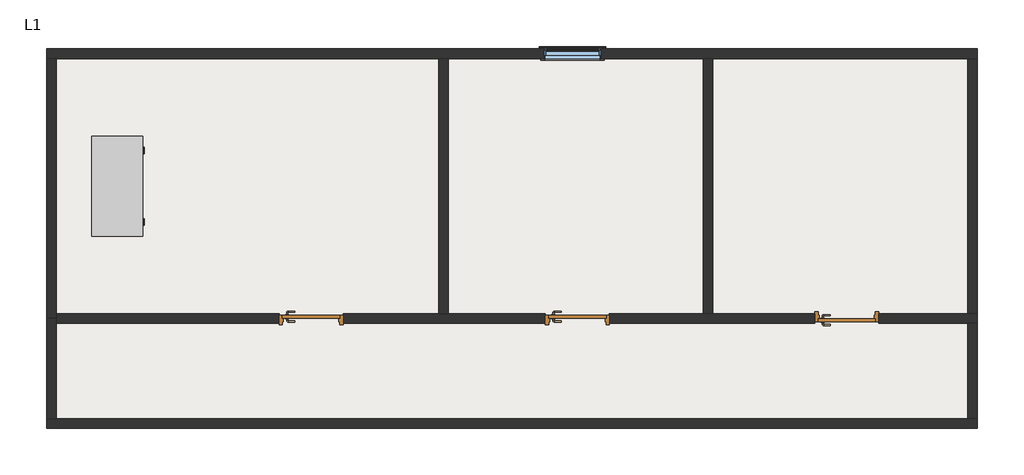
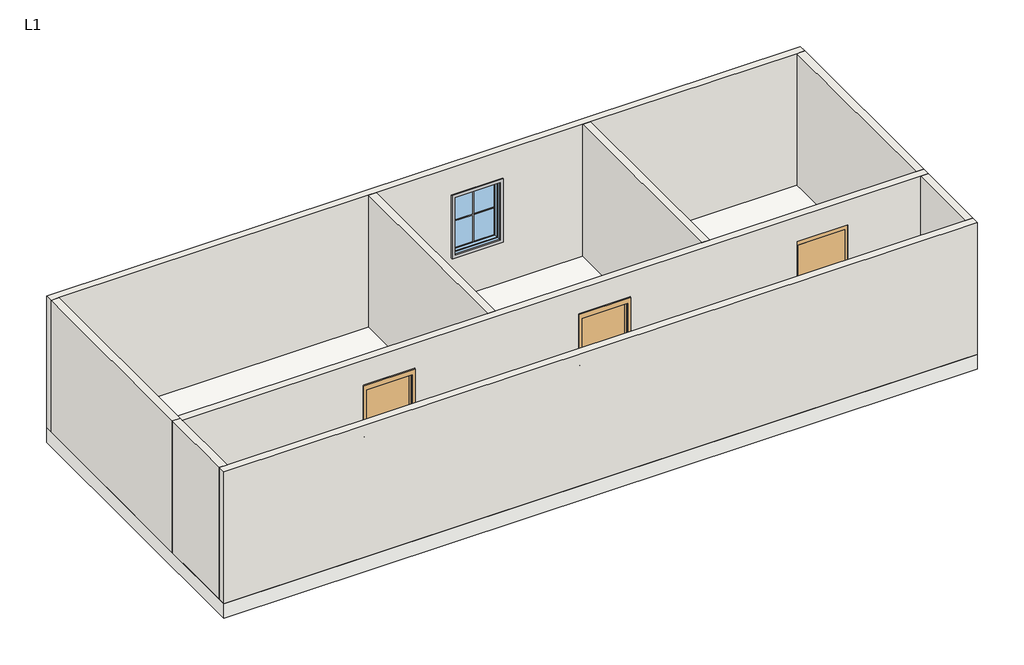
# One storey: 9 walls, 3 doors, 3 proxies, 1 furniture element, 1 slab, 1 window.
"""IFC4 building model written with IfcOpenShell, lengths in millimetres."""

import ifcopenshell
import ifcopenshell.guid

model = None  # the IFC model being written
_history = None  # IfcOwnerHistory: only IFC2X3 demands one
_inside = {}  # id of a spatial element -> (the spatial element, [elements in it])
_under = {}  # id of a project, library or spatial element -> (it, [spatial elements below it])
_declared = {}  # id of a project -> (the project, [libraries it declares])
_typed = {}  # id of a type object -> (the type object, [elements of that type])
_made_of = {}  # id of a material, layer set ... -> (it, [elements and type objects made of it])


def new_model(schema):
    """Start an empty IFC model of exactly this schema.

    Asked for "IFC4X3", IfcOpenShell would pick the latest addendum, in which some entities
    have other attributes; the version numbers below select the first issue.
    IFC2X3 requires an IfcOwnerHistory on every rooted entity: one is made here for all.
    """
    global model, _history
    if schema == "IFC4X3":
        model = ifcopenshell.file(schema_version=(4, 3, 0, 0))
    else:
        model = ifcopenshell.file(schema=schema)
    _inside.clear()
    _under.clear()
    _declared.clear()
    _typed.clear()
    _made_of.clear()
    _history = None
    if model.schema == "IFC2X3":
        org = make("IfcOrganization", Name="unknown")
        user = make(
            "IfcPersonAndOrganization",
            ThePerson=make("IfcPerson", FamilyName="unknown"),
            TheOrganization=org,
        )
        app = make(
            "IfcApplication",
            ApplicationDeveloper=org,
            Version="unknown",
            ApplicationFullName="unknown",
            ApplicationIdentifier="unknown",
        )
        _history = make(
            "IfcOwnerHistory",
            OwningUser=user,
            OwningApplication=app,
            ChangeAction="ADDED",
            CreationDate=0,
        )
    return model


def make(cls, **values):
    """One entity of the class cls with the attributes given. An attribute that is None is left unset."""
    return model.create_entity(
        cls, **{name: value for name, value in values.items() if value is not None}
    )


def rooted(cls, **values):
    """An entity with a GlobalId (a new one), such as an element, a storey or a relation."""
    return make(cls, GlobalId=ifcopenshell.guid.new(), OwnerHistory=_history, **values)


def si_unit(unit_type, name, prefix=None):
    """IfcSIUnit, for example si_unit("LENGTHUNIT", "METRE", prefix="MILLI")."""
    return make("IfcSIUnit", UnitType=unit_type, Prefix=prefix, Name=name)


def assignment(units):
    """IfcUnitAssignment: the units of a project."""
    return None if units is None else make("IfcUnitAssignment", Units=units)


def point(xyz):
    """IfcCartesianPoint."""
    return None if xyz is None else make("IfcCartesianPoint", Coordinates=xyz)


def direction(xyz):
    """IfcDirection."""
    return None if xyz is None else make("IfcDirection", DirectionRatios=xyz)


def frame(location, z_axis=None, x_axis=None):
    """IfcAxis2Placement3D, a coordinate frame: its origin and axes. An axis left out is left unset."""
    return make(
        "IfcAxis2Placement3D",
        Location=point(location),
        Axis=direction(z_axis),
        RefDirection=direction(x_axis),
    )


def frame_2d(location, x_axis=None):
    """IfcAxis2Placement2D, a coordinate frame in the plane: its origin and x axis."""
    return make(
        "IfcAxis2Placement2D", Location=point(location), RefDirection=direction(x_axis)
    )


def origin():
    """The frame at (0, 0, 0) with its axes left unset."""
    return frame((0.0, 0.0, 0.0))


def origin_with_axes():
    """The frame at (0, 0, 0) with the z axis (0, 0, 1) and the x axis (1, 0, 0) written out."""
    return frame((0.0, 0.0, 0.0), z_axis=(0.0, 0.0, 1.0), x_axis=(1.0, 0.0, 0.0))


def place(relative_to, where):
    """IfcLocalPlacement: puts the frame where relative to a parent placement (None: the world)."""
    return make(
        "IfcLocalPlacement", PlacementRelTo=relative_to, RelativePlacement=where
    )


def context(
    kind, dimensions, precision=None, world=None, true_north=None, identifier=None
):
    """IfcGeometricRepresentationContext, for example the 3D "Model" context."""
    return make(
        "IfcGeometricRepresentationContext",
        ContextIdentifier=identifier,
        ContextType=kind,
        CoordinateSpaceDimension=dimensions,
        Precision=precision,
        WorldCoordinateSystem=world,
        TrueNorth=true_north,
    )


def project(units=None, contexts=None):
    """IfcProject with its units and contexts."""
    return rooted(
        "IfcProject",
        Name="project",
        RepresentationContexts=contexts,
        UnitsInContext=assignment(units),
    )


def spatial(cls, under=None, at=None, **own):
    """A site, building, storey or space (cls), placed at a placement, below another one or the project."""
    s = rooted(cls, ObjectPlacement=at, **own)
    if under is not None:
        _under.setdefault(under.id(), (under, []))[1].append(s)
    return s


def polyline(points):
    """IfcPolyline through the points."""
    return make("IfcPolyline", Points=[point(p) for p in points])


def circle_curve(where, radius):
    """IfcCircle in the frame where."""
    return make("IfcCircle", Position=where, Radius=radius)


def ellipse_curve(where, semi_axis1, semi_axis2):
    """IfcEllipse in the frame where."""
    return make(
        "IfcEllipse", Position=where, SemiAxis1=semi_axis1, SemiAxis2=semi_axis2
    )


def trimmed(basis, trim1, trim2, sense, master):
    """IfcTrimmedCurve: the piece of a basis curve between two trims."""
    return make(
        "IfcTrimmedCurve",
        BasisCurve=basis,
        Trim1=trim1,
        Trim2=trim2,
        SenseAgreement=sense,
        MasterRepresentation=master,
    )


def segment(curve, same_sense, transition):
    """IfcCompositeCurveSegment."""
    return make(
        "IfcCompositeCurveSegment",
        Transition=transition,
        SameSense=same_sense,
        ParentCurve=curve,
    )


def composite_curve(segments, self_intersect=None):
    """IfcCompositeCurve: segments joined end to end."""
    return make("IfcCompositeCurve", Segments=segments, SelfIntersect=self_intersect)


def outline(outer, holes=None, kind="AREA"):
    """IfcArbitraryClosedProfileDef: a profile drawn as a closed curve; with holes, ...WithVoids."""
    if holes is None:
        return make("IfcArbitraryClosedProfileDef", ProfileType=kind, OuterCurve=outer)
    return make(
        "IfcArbitraryProfileDefWithVoids",
        ProfileType=kind,
        OuterCurve=outer,
        InnerCurves=holes,
    )


def extrude(swept, where, along, depth):
    """IfcExtrudedAreaSolid: the profile swept, set in the frame where, extruded along a direction by depth."""
    return make(
        "IfcExtrudedAreaSolid",
        SweptArea=swept,
        Position=where,
        ExtrudedDirection=direction(along),
        Depth=depth,
    )


def faces_of(points, faces, orient=None, outer=None):
    """IfcFace entities. A face is a list of loops; a loop is a list of indices into points, from 0.

    orient and outer hold one flag for each loop. By default every Orientation is true, the
    first loop of a face is its IfcFaceOuterBound and the others are IfcFaceBound.
    """
    made = []
    for i, loops in enumerate(faces):
        bounds = []
        for j, loop in enumerate(loops):
            is_outer = j == 0 if outer is None else outer[i][j]
            bounds.append(
                make(
                    "IfcFaceOuterBound" if is_outer else "IfcFaceBound",
                    Bound=make("IfcPolyLoop", Polygon=[points[k] for k in loop]),
                    Orientation=True if orient is None else orient[i][j],
                )
            )
        made.append(make("IfcFace", Bounds=bounds))
    return made


def faceted_brep(points, faces, orient=None, outer=None, voids=None):
    """IfcFacetedBrep: a solid bounded by flat faces; with voids (closed shells), ...WithVoids."""
    shared = [point(p) for p in points]
    hull = make("IfcClosedShell", CfsFaces=faces_of(shared, faces, orient, outer))
    if voids is None:
        return make("IfcFacetedBrep", Outer=hull)
    return make(
        "IfcFacetedBrepWithVoids",
        Outer=hull,
        Voids=[
            make(cls, CfsFaces=faces_of(shared, fs, o, b)) for cls, fs, o, b in voids
        ],
    )


def shape(context_of_items, identifier, shape_type, items):
    """IfcShapeRepresentation: the items that make up one representation, for example the "Body"."""
    return make(
        "IfcShapeRepresentation",
        ContextOfItems=context_of_items,
        RepresentationIdentifier=identifier,
        RepresentationType=shape_type,
        Items=items,
    )


def source(mapping_origin, context_of_items, identifier, shape_type, items):
    """IfcRepresentationMap: a shape defined once, which mapped items show again and again."""
    return make(
        "IfcRepresentationMap",
        MappingOrigin=mapping_origin,
        MappedRepresentation=shape(context_of_items, identifier, shape_type, items),
    )


def transform(
    local_origin,
    x_axis=None,
    y_axis=None,
    z_axis=None,
    scale=None,
    scale2=None,
    scale3=None,
    uniform=True,
):
    """IfcCartesianTransformationOperator3D, or its non-uniform kind. x_axis, y_axis, z_axis: its Axis1, 2, 3."""
    if uniform:
        return make(
            "IfcCartesianTransformationOperator3D",
            Axis1=direction(x_axis),
            Axis2=direction(y_axis),
            LocalOrigin=point(local_origin),
            Scale=scale,
            Axis3=direction(z_axis),
        )
    return make(
        "IfcCartesianTransformationOperator3DnonUniform",
        Axis1=direction(x_axis),
        Axis2=direction(y_axis),
        LocalOrigin=point(local_origin),
        Scale=scale,
        Axis3=direction(z_axis),
        Scale2=scale2,
        Scale3=scale3,
    )


def mapped(mapping_source, mapping_target):
    """IfcMappedItem: shows the shape of a source again, moved by a transform."""
    return make(
        "IfcMappedItem", MappingSource=mapping_source, MappingTarget=mapping_target
    )


def made_of(thing, what):
    """Note that an element or type object is made of a material, layer set ...; save() writes the relation."""
    if what is not None:
        _made_of.setdefault(what.id(), (what, []))[1].append(thing)
    return thing


def element(
    cls,
    number,
    at=None,
    inside=None,
    cuts=None,
    type_object=None,
    material=None,
    context=None,
    identifier="Body",
    shape_type=None,
    held_by="IfcProductDefinitionShape",
    body=None,
    shapes=None,
    **own,
):
    """One element of the class cls, such as IfcWall. Its Tag is "e" and its number.

    at: its placement. inside: the storey or other place that contains it. cuts: it is an
    opening in that element (IfcRelVoidsElement). A single representation is given by context,
    identifier, shape_type and body (its items); several are given by shapes. held_by: the class
    of the entity that holds the representations. save() writes the other relations.
    """
    e = rooted(cls, Tag="e%d" % number, ObjectPlacement=at, **own)
    if body is not None:
        shapes = [shape(context, identifier, shape_type, body)]
    if shapes is not None:
        e.Representation = make(held_by, Representations=shapes)
    if inside is not None:
        _inside.setdefault(inside.id(), (inside, []))[1].append(e)
    if cuts is not None:
        rooted(
            "IfcRelVoidsElement", RelatingBuildingElement=cuts, RelatedOpeningElement=e
        )
    if type_object is not None:
        _typed.setdefault(type_object.id(), (type_object, []))[1].append(e)
    return made_of(e, material)


def aggregate(whole, parts):
    """IfcRelAggregates: a whole, such as a stair, and the parts it consists of."""
    return rooted("IfcRelAggregates", RelatingObject=whole, RelatedObjects=parts)


def save(model, path):
    """Write the relations noted so far, then the file.

    IfcRelAggregates (storeys below a building ...), IfcRelContainedInSpatialStructure (elements
    in a storey), IfcRelDefinesByType, IfcRelAssociatesMaterial and IfcRelDeclares: one each for
    every whole, place, type object, material and project.
    """
    for whole, parts in _under.values():
        aggregate(whole, parts)
    for where, things in _inside.values():
        rooted(
            "IfcRelContainedInSpatialStructure",
            RelatedElements=things,
            RelatingStructure=where,
        )
    for kind, things in _typed.values():
        rooted("IfcRelDefinesByType", RelatedObjects=things, RelatingType=kind)
    for what, things in _made_of.values():
        rooted("IfcRelAssociatesMaterial", RelatedObjects=things, RelatingMaterial=what)
    for by, libraries in _declared.values():
        rooted("IfcRelDeclares", RelatingContext=by, RelatedDefinitions=libraries)
    model.write(path)


def plane_surface(at):
    """IfcPlane: the flat surface through the origin of the frame at, square to its z axis."""
    return make("IfcPlane", Position=at)


def cylinder_surface(at, radius):
    """IfcCylindricalSurface: all points at the distance radius from the z axis of the frame at."""
    return make("IfcCylindricalSurface", Position=at, Radius=radius)


def revolved_surface(curve, axis_point, axis_direction):
    """IfcSurfaceOfRevolution: the curve turned about the line through axis_point along axis_direction."""
    return make(
        "IfcSurfaceOfRevolution",
        SweptCurve=make("IfcArbitraryOpenProfileDef", ProfileType="CURVE", Curve=curve),
        AxisPosition=make("IfcAxis1Placement", Location=point(axis_point), Axis=direction(axis_direction)),
    )


def advanced_brep(points, edges, surfaces, faces):
    """IfcAdvancedBrep: a solid bounded by faces that lie on surfaces and meet in shared edges.

    An edge is (start, end): straight between two places in points (the first is 0);
    or (start, end, curve); or (start, end, curve, False) where it runs against its curve.
    A face is (place in surfaces, loops), or (place, loops, False) where it looks against
    its surface's normal. A loop lists edges by number (the first is 1), with a minus sign
    where the edge is run from its end to its start. The first loop is the outer one.
    """
    corners = [point(p) for p in points]
    vertices = [make("IfcVertexPoint", VertexGeometry=c) for c in corners]
    made = []
    for start, end, *more in edges:
        made.append(
            make(
                "IfcEdgeCurve",
                EdgeStart=vertices[start],
                EdgeEnd=vertices[end],
                EdgeGeometry=more[0] if more else make("IfcPolyline", Points=[corners[start], corners[end]]),
                SameSense=more[1] if len(more) > 1 else True,
            )
        )
    hull = []
    for where, loops, *sense in faces:
        bounds = []
        for j, loop in enumerate(loops):
            ring = [make("IfcOrientedEdge", EdgeElement=made[abs(k) - 1], Orientation=k > 0) for k in loop]
            bounds.append(
                make(
                    "IfcFaceOuterBound" if j == 0 else "IfcFaceBound",
                    Bound=make("IfcEdgeLoop", EdgeList=ring),
                    Orientation=True,
                )
            )
        hull.append(make("IfcAdvancedFace", Bounds=bounds, FaceSurface=surfaces[where], SameSense=sense[0] if sense else True))
    return make("IfcAdvancedBrep", Outer=make("IfcClosedShell", CfsFaces=hull))


def m_muntin_pattern_2x2_m_muntin_pattern_2x2_ad852c99(model_context):
    return source(origin(), model_context, "Body", "SweptSolid", [
        extrude(outline(polyline([(568.25, -6.35), (568.25, -411.9), (555.55, -411.9), (555.55, -6.35), (0.0, -6.35), (0.0, 6.35), (555.55, 6.35), (555.55, 411.9), (568.25, 411.9), (568.25, 6.35), (1123.8, 6.35), (1123.8, -6.35), (568.25, -6.35)])), frame((0.0, -22.225, 0.0), z_axis=(0.0, 1.0, 0.0), x_axis=(0.0, 0.0, 1.0)), (0.0, 0.0, 1.0), 12.7),
        extrude(outline(polyline([(568.25, -6.35), (568.25, -411.9), (555.55, -411.9), (555.55, -6.35), (0.0, -6.35), (0.0, 6.35), (555.55, 6.35), (555.55, 411.9), (568.25, 411.9), (568.25, 6.35), (1123.8, 6.35), (1123.8, -6.35), (568.25, -6.35)])), frame((0.0, 9.525, 0.0), z_axis=(0.0, 1.0, 0.0), x_axis=(0.0, 0.0, 1.0)), (0.0, 0.0, 1.0), 12.7),
    ])


def m_trim_window_exterior_flat_with_sill_71544b40(model_context):
    return source(origin(), model_context, "Body", "SweptSolid", [
        extrude(outline(polyline([(510.0, -1220.4323709), (510.0, -1280.4323709), (-510.0, -1280.4323709), (-510.0, -1220.4323709), (510.0, -1220.4323709)])), origin_with_axes(), (0.0, 0.0, 1.0), 19.05),
        extrude(outline(polyline([(-1230.0, 38.1), (-1202.4580645, 38.1), (-1200.0, 19.05), (-1200.0, 0.0), (-1220.4323709, 0.0), (-1220.4323709, 19.05), (-1230.0, 19.05), (-1230.0, 38.1)])), frame((-522.7, 0.0, 0.0), z_axis=(1.0, 0.0, 0.0), x_axis=(0.0, 1.0, 0.0)), (0.0, 0.0, 1.0), 1045.4),
        extrude(outline(polyline([(-510.0, 60.0), (510.0, 60.0), (510.0, -1200.0), (450.0, -1200.0), (450.0, 0.0), (-450.0, 0.0), (-450.0, -1200.0), (-510.0, -1200.0), (-510.0, 60.0)])), origin_with_axes(), (0.0, 0.0, 1.0), 19.05),
    ])


def m_trim_window_interior_flat_picture_frame_24fe8ef8(model_context):
    return source(origin(), model_context, "Body", "SweptSolid", [
        extrude(outline(polyline([(497.3, 47.3), (497.3, -1247.3), (-497.3, -1247.3), (-497.3, 47.3), (497.3, 47.3)]), holes=[polyline([(437.3, -12.7), (-437.3, -12.7), (-437.3, -1187.3), (437.3, -1187.3), (437.3, -12.7)])]), origin_with_axes(), (0.0, 0.0, 1.0), 30.0),
    ])


def m_door_passage_single_flush_900_x_2100mm_f70d95c9(model_context):
    return source(origin(), model_context, "Body", "SolidModel", [
        advanced_brep(
        [(-384.990625, 3.35, 1000.0), (-364.990625, 3.35, 1000.0), (-364.990625, -26.65, 1000.0), (-384.990625, -26.65, 1000.0), (-359.990625, -31.65, 1000.0), (-359.990625, -51.65, 1000.0), (-254.990625, -51.65, 1000.0), (-254.990625, -31.65, 1000.0)],
        [
            (0, 1, circle_curve(frame((-374.990625, 3.35, 1000.0), z_axis=(0.0, 1.0, 0.0), x_axis=(1.0, 0.0, 0.0)), 10.0)),
            (1, 0, circle_curve(frame((-374.990625, 3.35, 1000.0), z_axis=(0.0, 1.0, 0.0), x_axis=(1.0, 0.0, 0.0)), 10.0)),
            (1, 2),
            (2, 3, circle_curve(frame((-374.990625, -26.65, 1000.0), z_axis=(0.0, 1.0, 0.0), x_axis=(1.0, 0.0, 0.0)), 10.0)),
            (3, 0),
            (3, 2, circle_curve(frame((-374.990625, -26.65, 1000.0), z_axis=(0.0, 1.0, 0.0), x_axis=(1.0, 0.0, 0.0)), 10.0)),
            (4, 5, circle_curve(frame((-359.990625, -41.65, 1000.0), z_axis=(-1.0, 0.0, 0.0), x_axis=(0.0, 1.0, 0.0)), 10.0)),
            (5, 3, circle_curve(frame((-359.990625, -26.65, 1000.0), z_axis=(0.0, 0.0, -1.0), x_axis=(-1.0, 0.0, 0.0)), 25.0)),
            (2, 4, circle_curve(frame((-359.990625, -26.65, 1000.0), z_axis=(0.0, 0.0, 1.0), x_axis=(-1.0, 0.0, 0.0)), 5.0)),
            (5, 4, circle_curve(frame((-359.990625, -41.65, 1000.0), z_axis=(-1.0, 0.0, 0.0), x_axis=(0.0, 1.0, 0.0)), 10.0)),
            (6, 7, circle_curve(frame((-254.990625, -41.65, 1000.0), z_axis=(1.0, 0.0, 0.0), x_axis=(0.0, 1.0, 0.0)), 10.0)),
            (7, 6, circle_curve(frame((-254.990625, -41.65, 1000.0), z_axis=(1.0, 0.0, 0.0), x_axis=(0.0, 1.0, 0.0)), 10.0)),
            (4, 7),
            (6, 5),
        ],
        [
            plane_surface(frame((-374.990625, 3.35, 1000.0), z_axis=(0.0, 1.0, 0.0), x_axis=(0.0, 0.0, 1.0))),
            cylinder_surface(frame((-374.990625, 3.35, 1000.0), z_axis=(0.0, 1.0, 0.0), x_axis=(1.0, 0.0, 0.0)), 10.0),
            revolved_surface(trimmed(ellipse_curve(frame((-374.990625, -26.65, 1000.0), z_axis=(0.0, -1.0, 0.0), x_axis=(1.0, 0.0, 0.0)), 10.0, 10.0), [point((-384.990625, -26.65, 1000.0))], [point((-364.990625, -26.65, 1000.0))], True, "CARTESIAN"), (-359.990625, -26.65, 1000.0), (0.0, 0.0, -1.0)),
            revolved_surface(trimmed(ellipse_curve(frame((-374.990625, -26.65, 1000.0), z_axis=(0.0, -1.0, 0.0), x_axis=(1.0, 0.0, 0.0)), 10.0, 10.0), [point((-364.990625, -26.65, 1000.0))], [point((-384.990625, -26.65, 1000.0))], True, "CARTESIAN"), (-359.990625, -26.65, 1000.0), (0.0, 0.0, -1.0)),
            plane_surface(frame((-254.990625, -41.65, 1000.0), z_axis=(1.0, 0.0, 0.0), x_axis=(0.0, 0.0, 1.0))),
            cylinder_surface(frame((-359.990625, -41.65, 1000.0), z_axis=(-1.0, 0.0, 0.0), x_axis=(0.0, 1.0, 0.0)), 10.0),
        ],
        [
            (0, [[1, 2]]),
            (1, [[3, 4, 5, -2]]),
            (1, [[-5, 6, -3, -1]]),
            (2, [[7, 8, -4, 9]]),
            (3, [[10, -9, -6, -8]]),
            (4, [[11, 12]]),
            (5, [[13, -11, 14, -7]]),
            (5, [[-14, -12, -13, -10]]),
        ],
    ),
        extrude(outline(composite_curve([segment(trimmed(circle_curve(frame_2d((1000.0, -377.490625)), 30.0), [point((1000.0, -407.490625))], [point((1000.0, -347.490625))], False, "CARTESIAN"), True, "CONTINUOUS"), segment(trimmed(circle_curve(frame_2d((1000.0, -377.490625)), 30.0), [point((1000.0, -347.490625))], [point((1000.0, -407.490625))], False, "CARTESIAN"), True, "CONTINUOUS")], self_intersect=False)), frame((0.0, 3.35, 0.0), z_axis=(0.0, 1.0, 0.0), x_axis=(0.0, 0.0, 1.0)), (0.0, 0.0, 1.0), 8.0),
        advanced_brep(
        [(-384.990625, 64.35, 1000.0), (-364.990625, 64.35, 1000.0), (-384.990625, 94.35, 1000.0), (-364.990625, 94.35, 1000.0), (-359.990625, 99.35, 1000.0), (-359.990625, 119.35, 1000.0), (-254.990625, 119.35, 1000.0), (-254.990625, 99.35, 1000.0)],
        [
            (0, 1, circle_curve(frame((-374.990625, 64.35, 1000.0), z_axis=(0.0, -1.0, 0.0), x_axis=(1.0, 0.0, 0.0)), 10.0)),
            (1, 0, circle_curve(frame((-374.990625, 64.35, 1000.0), z_axis=(0.0, -1.0, 0.0), x_axis=(1.0, 0.0, 0.0)), 10.0)),
            (0, 2),
            (2, 3, circle_curve(frame((-374.990625, 94.35, 1000.0), z_axis=(0.0, -1.0, 0.0), x_axis=(1.0, 0.0, 0.0)), 10.0)),
            (3, 1),
            (3, 2, circle_curve(frame((-374.990625, 94.35, 1000.0), z_axis=(0.0, -1.0, 0.0), x_axis=(1.0, 0.0, 0.0)), 10.0)),
            (4, 3, circle_curve(frame((-359.990625, 94.35, 1000.0), z_axis=(0.0, 0.0, 1.0), x_axis=(-1.0, 0.0, 0.0)), 5.0)),
            (2, 5, circle_curve(frame((-359.990625, 94.35, 1000.0), z_axis=(0.0, 0.0, -1.0), x_axis=(-1.0, 0.0, 0.0)), 25.0)),
            (5, 4, circle_curve(frame((-359.990625, 109.35, 1000.0), z_axis=(-1.0, 0.0, 0.0), x_axis=(0.0, -1.0, 0.0)), 10.0)),
            (4, 5, circle_curve(frame((-359.990625, 109.35, 1000.0), z_axis=(-1.0, 0.0, 0.0), x_axis=(0.0, -1.0, 0.0)), 10.0)),
            (6, 7, circle_curve(frame((-254.990625, 109.35, 1000.0), z_axis=(1.0, 0.0, 0.0), x_axis=(0.0, -1.0, 0.0)), 10.0)),
            (7, 6, circle_curve(frame((-254.990625, 109.35, 1000.0), z_axis=(1.0, 0.0, 0.0), x_axis=(0.0, -1.0, 0.0)), 10.0)),
            (5, 6),
            (7, 4),
        ],
        [
            plane_surface(frame((-374.990625, 64.35, 1000.0), z_axis=(0.0, -1.0, 0.0), x_axis=(0.0, 0.0, 1.0))),
            cylinder_surface(frame((-374.990625, 64.35, 1000.0), z_axis=(0.0, -1.0, 0.0), x_axis=(1.0, 0.0, 0.0)), 10.0),
            revolved_surface(trimmed(ellipse_curve(frame((-374.990625, 94.35, 1000.0), z_axis=(0.0, -1.0, 0.0), x_axis=(1.0, 0.0, 0.0)), 10.0, 10.0), [point((-384.990625, 94.35, 1000.0))], [point((-364.990625, 94.35, 1000.0))], True, "CARTESIAN"), (-359.990625, 94.35, 1000.0), (0.0, 0.0, -1.0)),
            revolved_surface(trimmed(ellipse_curve(frame((-374.990625, 94.35, 1000.0), z_axis=(0.0, -1.0, 0.0), x_axis=(1.0, 0.0, 0.0)), 10.0, 10.0), [point((-364.990625, 94.35, 1000.0))], [point((-384.990625, 94.35, 1000.0))], True, "CARTESIAN"), (-359.990625, 94.35, 1000.0), (0.0, 0.0, -1.0)),
            plane_surface(frame((-254.990625, 109.35, 1000.0), z_axis=(1.0, 0.0, 0.0), x_axis=(0.0, 0.0, 1.0))),
            cylinder_surface(frame((-359.990625, 109.35, 1000.0), z_axis=(-1.0, 0.0, 0.0), x_axis=(0.0, -1.0, 0.0)), 10.0),
        ],
        [
            (0, [[1, 2]]),
            (1, [[-1, 3, 4, 5]]),
            (1, [[-2, -5, 6, -3]]),
            (2, [[7, -4, 8, 9]]),
            (3, [[-8, -6, -7, 10]]),
            (4, [[11, 12]]),
            (5, [[-9, 13, -12, 14]]),
            (5, [[-10, -14, -11, -13]]),
        ],
    ),
        extrude(outline(composite_curve([segment(trimmed(circle_curve(frame_2d((1000.0, -377.490625)), 30.0), [point((1000.0, -407.490625))], [point((1000.0, -347.490625))], False, "CARTESIAN"), True, "CONTINUOUS"), segment(trimmed(circle_curve(frame_2d((1000.0, -377.490625)), 30.0), [point((1000.0, -347.490625))], [point((1000.0, -407.490625))], False, "CARTESIAN"), True, "CONTINUOUS")], self_intersect=False)), frame((0.0, 56.35, 0.0), z_axis=(0.0, 1.0, 0.0), x_axis=(0.0, 0.0, 1.0)), (0.0, 0.0, 1.0), 8.0),
        extrude(outline(polyline([(450.0, 11.35), (-450.0, 11.35), (-450.0, 56.35), (450.0, 56.35), (450.0, 11.35)])), origin_with_axes(), (0.0, 0.0, 1.0), 2100.0),
        faceted_brep([(450.0, 6.5875, 0.0), (450.0, 56.35, 0.0), (500.0, 56.35, 0.0), (500.0, -93.65, 0.0), (450.0, -93.65, 0.0), (450.0, -44.4375, 0.0), (434.125, -44.4375, 0.0), (434.125, 6.5875, 0.0), (450.0, 6.5875, 2100.0), (450.0, 56.35, 2100.0), (-450.0, 56.35, 2100.0), (-450.0, 56.35, 0.0), (-500.0, 56.35, 0.0), (-500.0, 56.35, 2200.0), (500.0, 56.35, 2200.0), (500.0, -93.65, 2200.0), (-500.0, -93.65, 2200.0), (-500.0, -93.65, 0.0), (-450.0, -93.65, 0.0), (-450.0, -93.65, 2100.0), (450.0, -93.65, 2100.0), (450.0, -44.4375, 2100.0), (-450.0, -44.4375, 2100.0), (-450.0, -44.4375, 0.0), (-434.125, -44.4375, 0.0), (-434.125, -44.4375, 2084.125), (434.125, -44.4375, 2084.125), (434.125, 6.5875, 2084.125), (-434.125, 6.5875, 2084.125), (-434.125, 6.5875, 0.0), (-450.0, 6.5875, 0.0), (-450.0, 6.5875, 2100.0)], [[[0, 1, 2, 3, 4, 5, 6, 7]], [[1, 0, 8, 9]], [[2, 1, 9, 10, 11, 12, 13, 14]], [[3, 2, 14, 15]], [[4, 3, 15, 16, 17, 18, 19, 20]], [[5, 4, 20, 21]], [[6, 5, 21, 22, 23, 24, 25, 26]], [[7, 6, 26, 27]], [[0, 7, 27, 28, 29, 30, 31, 8]], [[9, 8, 31, 10]], [[20, 19, 22, 21]], [[26, 25, 28, 27]], [[12, 11, 30, 29, 24, 23, 18, 17]], [[11, 10, 31, 30]], [[13, 12, 17, 16]], [[19, 18, 23, 22]], [[25, 24, 29, 28]], [[15, 14, 13, 16]]]),
    ])


def m_door_passage_single_flush_900_x_2100mm_89322b7b(model_context):
    return source(origin(), model_context, "Body", "SolidModel", [
        advanced_brep(
        [(-384.990625, -3.35, 1000.0), (-364.990625, -3.35, 1000.0), (-384.990625, 26.65, 1000.0), (-364.990625, 26.65, 1000.0), (-359.990625, 31.65, 1000.0), (-359.990625, 51.65, 1000.0), (-254.990625, 51.65, 1000.0), (-254.990625, 31.65, 1000.0)],
        [
            (0, 1, circle_curve(frame((-374.990625, -3.35, 1000.0), z_axis=(0.0, -1.0, 0.0), x_axis=(1.0, 0.0, 0.0)), 10.0)),
            (1, 0, circle_curve(frame((-374.990625, -3.35, 1000.0), z_axis=(0.0, -1.0, 0.0), x_axis=(1.0, 0.0, 0.0)), 10.0)),
            (0, 2),
            (2, 3, circle_curve(frame((-374.990625, 26.65, 1000.0), z_axis=(0.0, -1.0, 0.0), x_axis=(1.0, 0.0, 0.0)), 10.0)),
            (3, 1),
            (3, 2, circle_curve(frame((-374.990625, 26.65, 1000.0), z_axis=(0.0, -1.0, 0.0), x_axis=(1.0, 0.0, 0.0)), 10.0)),
            (4, 3, circle_curve(frame((-359.990625, 26.65, 1000.0), z_axis=(0.0, 0.0, 1.0), x_axis=(-1.0, 0.0, 0.0)), 5.0)),
            (2, 5, circle_curve(frame((-359.990625, 26.65, 1000.0), z_axis=(0.0, 0.0, -1.0), x_axis=(-1.0, 0.0, 0.0)), 25.0)),
            (5, 4, circle_curve(frame((-359.990625, 41.65, 1000.0), z_axis=(-1.0, 0.0, 0.0), x_axis=(0.0, -1.0, 0.0)), 10.0)),
            (4, 5, circle_curve(frame((-359.990625, 41.65, 1000.0), z_axis=(-1.0, 0.0, 0.0), x_axis=(0.0, -1.0, 0.0)), 10.0)),
            (6, 7, circle_curve(frame((-254.990625, 41.65, 1000.0), z_axis=(1.0, 0.0, 0.0), x_axis=(0.0, -1.0, 0.0)), 10.0)),
            (7, 6, circle_curve(frame((-254.990625, 41.65, 1000.0), z_axis=(1.0, 0.0, 0.0), x_axis=(0.0, -1.0, 0.0)), 10.0)),
            (5, 6),
            (7, 4),
        ],
        [
            plane_surface(frame((-374.990625, -3.35, 1000.0), z_axis=(0.0, -1.0, 0.0), x_axis=(0.0, 0.0, 1.0))),
            cylinder_surface(frame((-374.990625, -3.35, 1000.0), z_axis=(0.0, -1.0, 0.0), x_axis=(1.0, 0.0, 0.0)), 10.0),
            revolved_surface(trimmed(ellipse_curve(frame((-374.990625, 26.65, 1000.0), z_axis=(0.0, -1.0, 0.0), x_axis=(1.0, 0.0, 0.0)), 10.0, 10.0), [point((-384.990625, 26.65, 1000.0))], [point((-364.990625, 26.65, 1000.0))], True, "CARTESIAN"), (-359.990625, 26.65, 1000.0), (0.0, 0.0, -1.0)),
            revolved_surface(trimmed(ellipse_curve(frame((-374.990625, 26.65, 1000.0), z_axis=(0.0, -1.0, 0.0), x_axis=(1.0, 0.0, 0.0)), 10.0, 10.0), [point((-364.990625, 26.65, 1000.0))], [point((-384.990625, 26.65, 1000.0))], True, "CARTESIAN"), (-359.990625, 26.65, 1000.0), (0.0, 0.0, -1.0)),
            plane_surface(frame((-254.990625, 41.65, 1000.0), z_axis=(1.0, 0.0, 0.0), x_axis=(0.0, 0.0, 1.0))),
            cylinder_surface(frame((-359.990625, 41.65, 1000.0), z_axis=(-1.0, 0.0, 0.0), x_axis=(0.0, -1.0, 0.0)), 10.0),
        ],
        [
            (0, [[1, 2]]),
            (1, [[-1, 3, 4, 5]]),
            (1, [[-2, -5, 6, -3]]),
            (2, [[7, -4, 8, 9]]),
            (3, [[-8, -6, -7, 10]]),
            (4, [[11, 12]]),
            (5, [[-9, 13, -12, 14]]),
            (5, [[-10, -14, -11, -13]]),
        ],
    ),
        extrude(outline(composite_curve([segment(trimmed(circle_curve(frame_2d((1000.0, -377.490625)), 30.0), [point((1000.0, -407.490625))], [point((1000.0, -347.490625))], False, "CARTESIAN"), True, "CONTINUOUS"), segment(trimmed(circle_curve(frame_2d((1000.0, -377.490625)), 30.0), [point((1000.0, -347.490625))], [point((1000.0, -407.490625))], False, "CARTESIAN"), True, "CONTINUOUS")], self_intersect=False)), frame((0.0, -11.35, 0.0), z_axis=(0.0, 1.0, 0.0), x_axis=(0.0, 0.0, 1.0)), (0.0, 0.0, 1.0), 8.0),
        advanced_brep(
        [(-384.990625, -64.35, 1000.0), (-364.990625, -64.35, 1000.0), (-364.990625, -94.35, 1000.0), (-384.990625, -94.35, 1000.0), (-359.990625, -99.35, 1000.0), (-359.990625, -119.35, 1000.0), (-254.990625, -119.35, 1000.0), (-254.990625, -99.35, 1000.0)],
        [
            (0, 1, circle_curve(frame((-374.990625, -64.35, 1000.0), z_axis=(0.0, 1.0, 0.0), x_axis=(1.0, 0.0, 0.0)), 10.0)),
            (1, 0, circle_curve(frame((-374.990625, -64.35, 1000.0), z_axis=(0.0, 1.0, 0.0), x_axis=(1.0, 0.0, 0.0)), 10.0)),
            (1, 2),
            (2, 3, circle_curve(frame((-374.990625, -94.35, 1000.0), z_axis=(0.0, 1.0, 0.0), x_axis=(1.0, 0.0, 0.0)), 10.0)),
            (3, 0),
            (3, 2, circle_curve(frame((-374.990625, -94.35, 1000.0), z_axis=(0.0, 1.0, 0.0), x_axis=(1.0, 0.0, 0.0)), 10.0)),
            (4, 5, circle_curve(frame((-359.990625, -109.35, 1000.0), z_axis=(-1.0, 0.0, 0.0), x_axis=(0.0, 1.0, 0.0)), 10.0)),
            (5, 3, circle_curve(frame((-359.990625, -94.35, 1000.0), z_axis=(0.0, 0.0, -1.0), x_axis=(-1.0, 0.0, 0.0)), 25.0)),
            (2, 4, circle_curve(frame((-359.990625, -94.35, 1000.0), z_axis=(0.0, 0.0, 1.0), x_axis=(-1.0, 0.0, 0.0)), 5.0)),
            (5, 4, circle_curve(frame((-359.990625, -109.35, 1000.0), z_axis=(-1.0, 0.0, 0.0), x_axis=(0.0, 1.0, 0.0)), 10.0)),
            (6, 7, circle_curve(frame((-254.990625, -109.35, 1000.0), z_axis=(1.0, 0.0, 0.0), x_axis=(0.0, 1.0, 0.0)), 10.0)),
            (7, 6, circle_curve(frame((-254.990625, -109.35, 1000.0), z_axis=(1.0, 0.0, 0.0), x_axis=(0.0, 1.0, 0.0)), 10.0)),
            (4, 7),
            (6, 5),
        ],
        [
            plane_surface(frame((-374.990625, -64.35, 1000.0), z_axis=(0.0, 1.0, 0.0), x_axis=(0.0, 0.0, 1.0))),
            cylinder_surface(frame((-374.990625, -64.35, 1000.0), z_axis=(0.0, 1.0, 0.0), x_axis=(1.0, 0.0, 0.0)), 10.0),
            revolved_surface(trimmed(ellipse_curve(frame((-374.990625, -94.35, 1000.0), z_axis=(0.0, -1.0, 0.0), x_axis=(1.0, 0.0, 0.0)), 10.0, 10.0), [point((-384.990625, -94.35, 1000.0))], [point((-364.990625, -94.35, 1000.0))], True, "CARTESIAN"), (-359.990625, -94.35, 1000.0), (0.0, 0.0, -1.0)),
            revolved_surface(trimmed(ellipse_curve(frame((-374.990625, -94.35, 1000.0), z_axis=(0.0, -1.0, 0.0), x_axis=(1.0, 0.0, 0.0)), 10.0, 10.0), [point((-364.990625, -94.35, 1000.0))], [point((-384.990625, -94.35, 1000.0))], True, "CARTESIAN"), (-359.990625, -94.35, 1000.0), (0.0, 0.0, -1.0)),
            plane_surface(frame((-254.990625, -109.35, 1000.0), z_axis=(1.0, 0.0, 0.0), x_axis=(0.0, 0.0, 1.0))),
            cylinder_surface(frame((-359.990625, -109.35, 1000.0), z_axis=(-1.0, 0.0, 0.0), x_axis=(0.0, 1.0, 0.0)), 10.0),
        ],
        [
            (0, [[1, 2]]),
            (1, [[3, 4, 5, -2]]),
            (1, [[-5, 6, -3, -1]]),
            (2, [[7, 8, -4, 9]]),
            (3, [[10, -9, -6, -8]]),
            (4, [[11, 12]]),
            (5, [[13, -11, 14, -7]]),
            (5, [[-14, -12, -13, -10]]),
        ],
    ),
        extrude(outline(composite_curve([segment(trimmed(circle_curve(frame_2d((1000.0, -377.490625)), 30.0), [point((1000.0, -407.490625))], [point((1000.0, -347.490625))], False, "CARTESIAN"), True, "CONTINUOUS"), segment(trimmed(circle_curve(frame_2d((1000.0, -377.490625)), 30.0), [point((1000.0, -347.490625))], [point((1000.0, -407.490625))], False, "CARTESIAN"), True, "CONTINUOUS")], self_intersect=False)), frame((0.0, -64.35, 0.0), z_axis=(0.0, 1.0, 0.0), x_axis=(0.0, 0.0, 1.0)), (0.0, 0.0, 1.0), 8.0),
        extrude(outline(polyline([(450.0, -11.35), (450.0, -56.35), (-450.0, -56.35), (-450.0, -11.35), (450.0, -11.35)])), origin_with_axes(), (0.0, 0.0, 1.0), 2100.0),
        faceted_brep([(450.0, -6.5875, 0.0), (434.125, -6.5875, 0.0), (434.125, 44.4375, 0.0), (450.0, 44.4375, 0.0), (450.0, 93.65, 0.0), (500.0, 93.65, 0.0), (500.0, -56.35, 0.0), (450.0, -56.35, 0.0), (450.0, -56.35, 2100.0), (450.0, -6.5875, 2100.0), (500.0, -56.35, 2200.0), (-500.0, -56.35, 2200.0), (-500.0, -56.35, 0.0), (-450.0, -56.35, 0.0), (-450.0, -56.35, 2100.0), (500.0, 93.65, 2200.0), (450.0, 93.65, 2100.0), (-450.0, 93.65, 2100.0), (-450.0, 93.65, 0.0), (-500.0, 93.65, 0.0), (-500.0, 93.65, 2200.0), (450.0, 44.4375, 2100.0), (434.125, 44.4375, 2084.125), (-434.125, 44.4375, 2084.125), (-434.125, 44.4375, 0.0), (-450.0, 44.4375, 0.0), (-450.0, 44.4375, 2100.0), (434.125, -6.5875, 2084.125), (-450.0, -6.5875, 2100.0), (-450.0, -6.5875, 0.0), (-434.125, -6.5875, 0.0), (-434.125, -6.5875, 2084.125)], [[[0, 1, 2, 3, 4, 5, 6, 7]], [[7, 8, 9, 0]], [[6, 10, 11, 12, 13, 14, 8, 7]], [[5, 15, 10, 6]], [[4, 16, 17, 18, 19, 20, 15, 5]], [[3, 21, 16, 4]], [[2, 22, 23, 24, 25, 26, 21, 3]], [[1, 27, 22, 2]], [[0, 9, 28, 29, 30, 31, 27, 1]], [[8, 14, 28, 9]], [[16, 21, 26, 17]], [[22, 27, 31, 23]], [[12, 19, 18, 25, 24, 30, 29, 13]], [[13, 29, 28, 14]], [[11, 20, 19, 12]], [[17, 26, 25, 18]], [[23, 31, 30, 24]], [[15, 20, 11, 10]]]),
    ])


def m_desk_1525_x_762mm_student_34485ced(model_context):
    return source(origin(), model_context, "Body", "SolidModel", [
        extrude(outline(polyline([(1118.1, 0.0), (1118.1, 635.0), (405.9, 635.0), (405.9, 0.0), (-0.5, 0.0), (-0.5, 762.0), (1524.5, 762.0), (1524.5, 0.0), (1118.1, 0.0)])), frame((0.0, 0.0, 152.0), z_axis=(0.0, 0.0, 1.0), x_axis=(1.0, 0.0, 0.0)), (0.0, 0.0, 1.0), 571.9),
        extrude(outline(polyline([(-19.55, -19.05), (-19.55, 781.05), (1543.55, 781.05), (1543.55, -19.05), (-19.55, -19.05)])), frame((0.0, 0.0, 723.9), z_axis=(0.0, 0.0, 1.0), x_axis=(1.0, 0.0, 0.0)), (0.0, 0.0, 1.0), 38.1),
        faceted_brep([(1422.9, 0.0, 152.0), (1524.5, 0.0, 152.0), (1524.5, 101.6, 152.0), (1422.9, 101.6, 152.0), (1448.3, 0.0, 0.0), (1448.3, 76.2, 0.0), (1524.5, 76.2, 0.0), (1524.5, 0.0, 0.0)], [[[0, 1, 2, 3]], [[4, 5, 6, 7]], [[4, 7, 1, 0]], [[7, 6, 2, 1]], [[6, 5, 3, 2]], [[5, 4, 0, 3]]]),
        faceted_brep([(1422.9, 762.0, 152.0), (1422.9, 660.4, 152.0), (1524.5, 660.4, 152.0), (1524.5, 762.0, 152.0), (1448.3, 762.0, 0.0), (1524.5, 762.0, 0.0), (1524.5, 685.8, 0.0), (1448.3, 685.8, 0.0)], [[[0, 1, 2, 3]], [[4, 5, 6, 7]], [[4, 7, 1, 0]], [[7, 6, 2, 1]], [[6, 5, 3, 2]], [[5, 4, 0, 3]]]),
        faceted_brep([(101.1, 762.0, 152.0), (-0.5, 762.0, 152.0), (-0.5, 660.4, 152.0), (101.1, 660.4, 152.0), (75.7, 762.0, 0.0), (75.7, 685.8, 0.0), (-0.5, 685.8, 0.0), (-0.5, 762.0, 0.0)], [[[0, 1, 2, 3]], [[4, 5, 6, 7]], [[4, 7, 1, 0]], [[7, 6, 2, 1]], [[6, 5, 3, 2]], [[5, 4, 0, 3]]]),
        faceted_brep([(101.1, 0.0, 152.0), (101.1, 101.6, 152.0), (-0.5, 101.6, 152.0), (-0.5, 0.0, 152.0), (75.7, 0.0, 0.0), (-0.5, 0.0, 0.0), (-0.5, 76.2, 0.0), (75.7, 76.2, 0.0)], [[[0, 1, 2, 3]], [[4, 5, 6, 7]], [[4, 7, 1, 0]], [[7, 6, 2, 1]], [[6, 5, 3, 2]], [[5, 4, 0, 3]]]),
        extrude(outline(polyline([(1137.15, 0.0), (1505.45, 0.0), (1505.45, -12.7), (1137.15, -12.7), (1137.15, 0.0)])), frame((0.0, 0.0, 602.85), z_axis=(0.0, 0.0, 1.0), x_axis=(1.0, 0.0, 0.0)), (0.0, 0.0, 1.0), 102.0),
        extrude(outline(polyline([(1137.15, 0.0), (1505.45, 0.0), (1505.45, -12.7), (1137.15, -12.7), (1137.15, 0.0)])), frame((0.0, 0.0, 171.05), z_axis=(0.0, 0.0, 1.0), x_axis=(1.0, 0.0, 0.0)), (0.0, 0.0, 1.0), 171.45),
        extrude(outline(polyline([(1137.15, 0.0), (1505.45, 0.0), (1505.45, -12.7), (1137.15, -12.7), (1137.15, 0.0)])), frame((0.0, 0.0, 482.2), z_axis=(0.0, 0.0, 1.0), x_axis=(1.0, 0.0, 0.0)), (0.0, 0.0, 1.0), 101.6),
        extrude(outline(polyline([(1137.15, 0.0), (1505.45, 0.0), (1505.45, -12.7), (1137.15, -12.7), (1137.15, 0.0)])), frame((0.0, 0.0, 361.55), z_axis=(0.0, 0.0, 1.0), x_axis=(1.0, 0.0, 0.0)), (0.0, 0.0, 1.0), 101.6),
        extrude(outline(polyline([(18.55, 0.0), (386.85, 0.0), (386.85, -12.7), (18.55, -12.7), (18.55, 0.0)])), frame((0.0, 0.0, 603.25), z_axis=(0.0, 0.0, 1.0), x_axis=(1.0, 0.0, 0.0)), (0.0, 0.0, 1.0), 101.6),
        extrude(outline(polyline([(18.55, 0.0), (386.85, 0.0), (386.85, -12.7), (18.55, -12.7), (18.55, 0.0)])), frame((0.0, 0.0, 171.05), z_axis=(0.0, 0.0, 1.0), x_axis=(1.0, 0.0, 0.0)), (0.0, 0.0, 1.0), 413.15),
        faceted_brep([(1365.75, -12.7, 304.8), (1372.1, -12.7, 304.8), (1372.1, -12.7, 292.1), (1365.75, -12.7, 292.1), (1365.75, -31.75, 304.8), (1372.1, -38.1, 304.8), (1372.1, -38.1, 292.1), (1365.75, -31.75, 292.1), (1276.85, -31.75, 304.8), (1270.5, -38.1, 304.8), (1270.5, -38.1, 292.1), (1276.85, -31.75, 292.1), (1276.85, -12.7, 304.8), (1276.85, -12.7, 292.1), (1270.5, -12.7, 292.1), (1270.5, -12.7, 304.8)], [[[0, 1, 2, 3]], [[1, 0, 4, 5]], [[2, 1, 5, 6]], [[3, 2, 6, 7]], [[0, 3, 7, 4]], [[5, 4, 8, 9]], [[6, 5, 9, 10]], [[7, 6, 10, 11]], [[4, 7, 11, 8]], [[12, 13, 14, 15]], [[9, 8, 12, 15]], [[10, 9, 15, 14]], [[11, 10, 14, 13]], [[8, 11, 13, 12]]]),
        faceted_brep([(1365.75, -12.7, 425.45), (1372.1, -12.7, 425.45), (1372.1, -12.7, 412.75), (1365.75, -12.7, 412.75), (1365.75, -31.75, 425.45), (1372.1, -38.1, 425.45), (1372.1, -38.1, 412.75), (1365.75, -31.75, 412.75), (1276.85, -31.75, 425.45), (1270.5, -38.1, 425.45), (1270.5, -38.1, 412.75), (1276.85, -31.75, 412.75), (1276.85, -12.7, 425.45), (1276.85, -12.7, 412.75), (1270.5, -12.7, 412.75), (1270.5, -12.7, 425.45)], [[[0, 1, 2, 3]], [[1, 0, 4, 5]], [[2, 1, 5, 6]], [[3, 2, 6, 7]], [[0, 3, 7, 4]], [[5, 4, 8, 9]], [[6, 5, 9, 10]], [[7, 6, 10, 11]], [[4, 7, 11, 8]], [[12, 13, 14, 15]], [[9, 8, 12, 15]], [[10, 9, 15, 14]], [[11, 10, 14, 13]], [[8, 11, 13, 12]]]),
        faceted_brep([(1365.75, -12.7, 546.1), (1372.1, -12.7, 546.1), (1372.1, -12.7, 533.4), (1365.75, -12.7, 533.4), (1365.75, -31.75, 546.1), (1372.1, -38.1, 546.1), (1372.1, -38.1, 533.4), (1365.75, -31.75, 533.4), (1276.85, -31.75, 546.1), (1270.5, -38.1, 546.1), (1270.5, -38.1, 533.4), (1276.85, -31.75, 533.4), (1276.85, -12.7, 546.1), (1276.85, -12.7, 533.4), (1270.5, -12.7, 533.4), (1270.5, -12.7, 546.1)], [[[0, 1, 2, 3]], [[1, 0, 4, 5]], [[2, 1, 5, 6]], [[3, 2, 6, 7]], [[0, 3, 7, 4]], [[5, 4, 8, 9]], [[6, 5, 9, 10]], [[7, 6, 10, 11]], [[4, 7, 11, 8]], [[12, 13, 14, 15]], [[9, 8, 12, 15]], [[10, 9, 15, 14]], [[11, 10, 14, 13]], [[8, 11, 13, 12]]]),
        faceted_brep([(1365.75, -12.7, 666.75), (1372.1, -12.7, 666.75), (1372.1, -12.7, 654.05), (1365.75, -12.7, 654.05), (1365.75, -31.75, 666.75), (1372.1, -38.1, 666.75), (1372.1, -38.1, 654.05), (1365.75, -31.75, 654.05), (1276.85, -31.75, 666.75), (1270.5, -38.1, 666.75), (1270.5, -38.1, 654.05), (1276.85, -31.75, 654.05), (1276.85, -12.7, 666.75), (1276.85, -12.7, 654.05), (1270.5, -12.7, 654.05), (1270.5, -12.7, 666.75)], [[[0, 1, 2, 3]], [[1, 0, 4, 5]], [[2, 1, 5, 6]], [[3, 2, 6, 7]], [[0, 3, 7, 4]], [[5, 4, 8, 9]], [[6, 5, 9, 10]], [[7, 6, 10, 11]], [[4, 7, 11, 8]], [[12, 13, 14, 15]], [[9, 8, 12, 15]], [[10, 9, 15, 14]], [[11, 10, 14, 13]], [[8, 11, 13, 12]]]),
        faceted_brep([(158.25, -12.7, 546.1), (158.25, -12.7, 533.4), (151.9, -12.7, 533.4), (151.9, -12.7, 546.1), (158.25, -31.75, 546.1), (158.25, -31.75, 533.4), (151.9, -38.1, 533.4), (151.9, -38.1, 546.1), (247.15, -31.75, 546.1), (247.15, -31.75, 533.4), (253.5, -38.1, 533.4), (253.5, -38.1, 546.1), (247.15, -12.7, 546.1), (253.5, -12.7, 546.1), (253.5, -12.7, 533.4), (247.15, -12.7, 533.4)], [[[0, 1, 2, 3]], [[1, 0, 4, 5]], [[2, 1, 5, 6]], [[3, 2, 6, 7]], [[0, 3, 7, 4]], [[5, 4, 8, 9]], [[6, 5, 9, 10]], [[7, 6, 10, 11]], [[4, 7, 11, 8]], [[12, 13, 14, 15]], [[9, 8, 12, 15]], [[10, 9, 15, 14]], [[11, 10, 14, 13]], [[8, 11, 13, 12]]]),
        faceted_brep([(158.25, -12.7, 666.75), (158.25, -12.7, 654.05), (151.9, -12.7, 654.05), (151.9, -12.7, 666.75), (158.25, -31.75, 666.75), (158.25, -31.75, 654.05), (151.9, -38.1, 654.05), (151.9, -38.1, 666.75), (247.15, -31.75, 666.75), (247.15, -31.75, 654.05), (253.5, -38.1, 654.05), (253.5, -38.1, 666.75), (247.15, -12.7, 666.75), (253.5, -12.7, 666.75), (253.5, -12.7, 654.05), (247.15, -12.7, 654.05)], [[[0, 1, 2, 3]], [[1, 0, 4, 5]], [[2, 1, 5, 6]], [[3, 2, 6, 7]], [[0, 3, 7, 4]], [[5, 4, 8, 9]], [[6, 5, 9, 10]], [[7, 6, 10, 11]], [[4, 7, 11, 8]], [[12, 13, 14, 15]], [[9, 8, 12, 15]], [[10, 9, 15, 14]], [[11, 10, 14, 13]], [[8, 11, 13, 12]]]),
    ])


def m_window_fixed_900_x_1200mm_f2c8dc95(model_context):
    return source(origin(), model_context, "Body", "SolidModel", [
        faceted_brep([(450.0, -20.25, 2100.0), (450.0, 94.05, 2100.0), (-450.0, 94.05, 2100.0), (-450.0, -20.25, 2100.0), (-450.0, 94.05, 900.0), (-450.0, -20.25, 900.0), (450.0, 94.05, 900.0), (450.0, -20.25, 900.0), (418.25, -20.25, 2068.25), (418.25, -20.25, 931.75), (-418.25, -20.25, 931.75), (-418.25, -20.25, 2068.25), (-437.3, 94.05, 2087.3), (-437.3, 94.05, 912.7), (437.3, 94.05, 912.7), (437.3, 94.05, 2087.3), (418.25, 43.25, 2068.25), (-418.25, 43.25, 2068.25), (437.3, 43.25, 2087.3), (-437.3, 43.25, 2087.3), (-418.25, 43.25, 931.75), (-437.3, 43.25, 912.7), (418.25, 43.25, 931.75), (437.3, 43.25, 912.7)], [[[0, 1, 2, 3]], [[3, 2, 4, 5]], [[5, 4, 6, 7]], [[3, 5, 7, 0], [8, 9, 10, 11]], [[7, 6, 1, 0]], [[1, 6, 4, 2], [12, 13, 14, 15]], [[16, 8, 11, 17]], [[15, 18, 19, 12]], [[17, 11, 10, 20]], [[12, 19, 21, 13]], [[20, 10, 9, 22]], [[13, 21, 23, 14]], [[22, 9, 8, 16]], [[18, 23, 21, 19], [17, 20, 22, 16]], [[14, 23, 18, 15]]]),
        extrude(outline(polyline([(2100.0, -450.0), (900.0, -450.0), (900.0, 450.0), (2100.0, 450.0), (2100.0, -450.0)]), holes=[polyline([(2087.3, 437.3), (912.7, 437.3), (912.7, -437.3), (2087.3, -437.3), (2087.3, 437.3)])]), frame((0.0, -75.0, 0.0), z_axis=(0.0, 1.0, 0.0), x_axis=(0.0, 0.0, 1.0)), (0.0, 0.0, 1.0), 54.75),
        extrude(outline(polyline([(912.7, 437.3), (2087.3, 437.3), (2087.3, -437.3), (912.7, -437.3), (912.7, 437.3)]), holes=[polyline([(938.1, -411.9), (2061.9, -411.9), (2061.9, 411.9), (938.1, 411.9), (938.1, -411.9)])]), frame((0.0, 43.25, 0.0), z_axis=(0.0, 1.0, 0.0), x_axis=(0.0, 0.0, 1.0)), (0.0, 0.0, 1.0), 44.45),
        extrude(outline(polyline([(411.9, 75.0), (411.9, 68.65), (-411.9, 68.65), (-411.9, 75.0), (411.9, 75.0)])), frame((0.0, 0.0, 938.1), z_axis=(0.0, 0.0, 1.0), x_axis=(1.0, 0.0, 0.0)), (0.0, 0.0, 1.0), 1123.8),
        extrude(outline(polyline([(-411.9, 55.95), (-411.9, 62.3), (411.9, 62.3), (411.9, 55.95), (-411.9, 55.95)])), frame((0.0, 0.0, 938.1), z_axis=(0.0, 0.0, 1.0), x_axis=(1.0, 0.0, 0.0)), (0.0, 0.0, 1.0), 1123.8),
    ])


model = new_model("IFC4")

# Units and contexts
model_context = context("Model", 3, world=origin())
ifc_project = project(units=[si_unit("LENGTHUNIT", "METRE", prefix="MILLI")], contexts=[model_context])

# Site, building, storey
site = spatial("IfcSite", under=ifc_project)
building = spatial("IfcBuilding", under=site)
storey = spatial("IfcBuildingStorey", under=building, Name="L1", Elevation=0.0)

# Proxies
placement = place(None, origin())
m_muntin_pattern_2x2_m_muntin_pattern_2x2_shape = m_muntin_pattern_2x2_m_muntin_pattern_2x2_ad852c99(model_context)
element("IfcBuildingElementProxy", 1, Name="M_Muntin Pattern_2x2 : M_Muntin Pattern_2x2", ObjectType="M_Muntin Pattern_2x2 : M_Muntin Pattern_2x2", at=placement, inside=storey, context=model_context, shape_type="MappedRepresentation", body=[
    mapped(m_muntin_pattern_2x2_m_muntin_pattern_2x2_shape, transform((1875.0, 4215.475, 938.1), x_axis=(-1.0, 0.0, 0.0), y_axis=(0.0, -1.0, 0.0), z_axis=(0.0, 0.0, 1.0))),
])
m_trim_window_exterior_flat_with_sill_shape = m_trim_window_exterior_flat_with_sill_71544b40(model_context)
element("IfcBuildingElementProxy", 2, Name="M_Trim-Window-Exterior-Flat : with Sill", ObjectType="M_Trim-Window-Exterior-Flat : with Sill", at=placement, inside=storey, context=model_context, shape_type="MappedRepresentation", body=[
    mapped(m_trim_window_exterior_flat_with_sill_shape, transform((1875.0, 4225.0, 2100.0), x_axis=(-1.0, 0.0, 0.0), y_axis=(0.0, 0.0, 1.0), z_axis=(0.0, 1.0, 0.0))),
])
m_trim_window_interior_flat_picture_frame_shape = m_trim_window_interior_flat_picture_frame_24fe8ef8(model_context)
element("IfcBuildingElementProxy", 3, Name="M_Trim-Window-Interior-Flat : Picture Frame", ObjectType="M_Trim-Window-Interior-Flat : Picture Frame", at=placement, inside=storey, context=model_context, shape_type="MappedRepresentation", body=[
    mapped(m_trim_window_interior_flat_picture_frame_shape, transform((1875.0, 4075.0, 2100.0), x_axis=(1.0, 0.0, 0.0), y_axis=(0.0, 0.0, 1.0), z_axis=(0.0, -1.0, 0.0))),
])

# Doors
m_door_passage_single_flush_900_x_2100mm_shape = m_door_passage_single_flush_900_x_2100mm_f70d95c9(model_context)
element("IfcDoor", 4, ObjectType="M_Door-Passage-Single-Flush : 900 x 2100mm", at=placement, inside=storey, context=model_context, shape_type="MappedRepresentation", body=[
    mapped(m_door_passage_single_flush_900_x_2100mm_shape, transform((1950.0, -6.35, 0.0), x_axis=(1.0, 0.0, 0.0), y_axis=(0.0, 1.0, 0.0), z_axis=(0.0, 0.0, 1.0))),
])
element("IfcDoor", 5, ObjectType="M_Door-Passage-Single-Flush : 900 x 2100mm", at=placement, inside=storey, context=model_context, shape_type="MappedRepresentation", body=[
    mapped(m_door_passage_single_flush_900_x_2100mm_shape, transform((-2225.0, -6.35, 0.0), x_axis=(1.0, 0.0, 0.0), y_axis=(0.0, 1.0, 0.0), z_axis=(0.0, 0.0, 1.0))),
])
m_door_passage_single_flush_900_x_2100mm_2_shape = m_door_passage_single_flush_900_x_2100mm_89322b7b(model_context)
element("IfcDoor", 6, ObjectType="M_Door-Passage-Single-Flush : 900 x 2100mm", at=placement, inside=storey, context=model_context, shape_type="MappedRepresentation", body=[
    mapped(m_door_passage_single_flush_900_x_2100mm_2_shape, transform((6175.0, 6.35, 0.0), x_axis=(1.0, 0.0, 0.0), y_axis=(0.0, 1.0, 0.0), z_axis=(0.0, 0.0, 1.0))),
])

# Furniture
m_desk_1525_x_762mm_student_shape = m_desk_1525_x_762mm_student_34485ced(model_context)
element("IfcFurniture", 7, ObjectType="M_Desk : 1525 x 762mm Student", at=placement, inside=storey, context=model_context, shape_type="MappedRepresentation", body=[
    mapped(m_desk_1525_x_762mm_student_shape, transform((-4883.0, 1310.5, 0.0), x_axis=(0.0, 1.0, 0.0), y_axis=(-1.0, 0.0, 0.0), z_axis=(0.0, 0.0, 1.0))),
])

# Slab
element("IfcSlab", 8, ObjectType="Generic 300mm", at=placement, inside=storey, context=model_context, shape_type="SweptSolid", body=[
    extrude(outline(polyline([(8225.0, 4225.0), (8225.0, -1725.0), (-6375.0, -1725.0), (-6375.0, 4225.0), (8225.0, 4225.0)])), frame((0.0, 0.0, -300.0), z_axis=(0.0, 0.0, 1.0), x_axis=(1.0, 0.0, 0.0)), (0.0, 0.0, 1.0), 300.0),
])

# Walls
element("IfcWall", 9, ObjectType="Generic - 150mm", at=placement, inside=storey, context=model_context, shape_type="SweptSolid", body=[
    extrude(outline(polyline([(-75.0, 4075.0), (-75.0, 75.0), (-225.0, 75.0), (-225.0, 4075.0), (-75.0, 4075.0)])), origin_with_axes(), (0.0, 0.0, 1.0), 2700.0),
])
element("IfcWall", 10, ObjectType="Generic - 150mm", at=placement, inside=storey, context=model_context, shape_type="Brep", body=[
    faceted_brep([(-6375.0, 4075.0, 0.0), (-6225.0, 4075.0, 0.0), (-225.0, 4075.0, 0.0), (-75.0, 4075.0, 0.0), (3925.0, 4075.0, 0.0), (4075.0, 4075.0, 0.0), (8075.0, 4075.0, 0.0), (8225.0, 4075.0, 0.0), (8225.0, 4075.0, 2700.0), (8075.0, 4075.0, 2700.0), (4075.0, 4075.0, 2700.0), (3925.0, 4075.0, 2700.0), (-75.0, 4075.0, 2700.0), (-225.0, 4075.0, 2700.0), (-6225.0, 4075.0, 2700.0), (-6375.0, 4075.0, 2700.0), (2325.0, 4075.0, 2100.0), (2325.0, 4075.0, 900.0), (1425.0, 4075.0, 900.0), (1425.0, 4075.0, 2100.0), (-6375.0, 4225.0, 0.0), (-6375.0, 4225.0, 2700.0), (8225.0, 4225.0, 2700.0), (8225.0, 4225.0, 0.0), (2325.0, 4225.0, 2100.0), (1425.0, 4225.0, 2100.0), (1425.0, 4225.0, 900.0), (2325.0, 4225.0, 900.0)], [[[0, 1, 2, 3, 4, 5, 6, 7, 8, 9, 10, 11, 12, 13, 14, 15], [16, 17, 18, 19]], [[20, 21, 22, 23], [24, 25, 26, 27]], [[7, 6, 5, 4, 3, 2, 1, 0, 20, 23]], [[15, 14, 13, 12, 11, 10, 9, 8, 22, 21]], [[0, 15, 21, 20]], [[8, 7, 23, 22]], [[17, 16, 24, 27]], [[18, 17, 27, 26]], [[19, 18, 26, 25]], [[16, 19, 25, 24]]]),
])
element("IfcWall", 11, ObjectType="Generic - 150mm", at=placement, inside=storey, context=model_context, shape_type="SweptSolid", body=[
    extrude(outline(polyline([(3925.0, 75.0), (3925.0, 4075.0), (4075.0, 4075.0), (4075.0, 75.0), (3925.0, 75.0)])), origin_with_axes(), (0.0, 0.0, 1.0), 2700.0),
])
element("IfcWall", 12, ObjectType="Generic - 150mm", at=placement, inside=storey, context=model_context, shape_type="SweptSolid", body=[
    extrude(outline(polyline([(-6375.0, 0.0), (-6375.0, 4075.0), (-6225.0, 4075.0), (-6225.0, 0.0), (-6375.0, 0.0)])), origin_with_axes(), (0.0, 0.0, 1.0), 2700.0),
])
element("IfcWall", 13, ObjectType="Generic - 150mm", at=placement, inside=storey, context=model_context, shape_type="SweptSolid", body=[
    extrude(outline(polyline([(8075.0, 75.0), (8075.0, 4075.0), (8225.0, 4075.0), (8225.0, 75.0), (8075.0, 75.0)])), origin_with_axes(), (0.0, 0.0, 1.0), 2700.0),
])
element("IfcWall", 14, ObjectType="Generic - 150mm", at=placement, inside=storey, context=model_context, shape_type="Brep", body=[
    faceted_brep([(8225.0, -1575.0, 0.0), (8075.0, -1575.0, 0.0), (-6225.0, -1575.0, 0.0), (-6375.0, -1575.0, 0.0), (-6375.0, -1575.0, 2700.0), (-6225.0, -1575.0, 2700.0), (8075.0, -1575.0, 2700.0), (8225.0, -1575.0, 2700.0), (8225.0, -1725.0, 0.0), (8225.0, -1725.0, 2700.0), (-6375.0, -1725.0, 2700.0), (-6375.0, -1725.0, 0.0)], [[[0, 1, 2, 3, 4, 5, 6, 7]], [[8, 9, 10, 11]], [[3, 2, 1, 0, 8, 11]], [[7, 6, 5, 4, 10, 9]], [[4, 3, 11, 10]], [[0, 7, 9, 8]]]),
])
element("IfcWall", 15, ObjectType="Generic - 150mm", at=placement, inside=storey, context=model_context, shape_type="Brep", body=[
    faceted_brep([(-6225.0, 75.0, 0.0), (-6225.0, 75.0, 2700.0), (-225.0, 75.0, 2700.0), (-75.0, 75.0, 2700.0), (3925.0, 75.0, 2700.0), (4075.0, 75.0, 2700.0), (8075.0, 75.0, 2700.0), (8225.0, 75.0, 2700.0), (8225.0, 75.0, 0.0), (8075.0, 75.0, 0.0), (6675.0, 75.0, 0.0), (6675.0, 75.0, 2200.0), (5675.0, 75.0, 2200.0), (5675.0, 75.0, 0.0), (4075.0, 75.0, 0.0), (3925.0, 75.0, 0.0), (2450.0, 75.0, 0.0), (2450.0, 75.0, 2200.0), (1450.0, 75.0, 2200.0), (1450.0, 75.0, 0.0), (-75.0, 75.0, 0.0), (-225.0, 75.0, 0.0), (-1725.0, 75.0, 0.0), (-1725.0, 75.0, 2200.0), (-2725.0, 75.0, 2200.0), (-2725.0, 75.0, 0.0), (-6225.0, -75.0, 2700.0), (-6225.0, -75.0, 0.0), (-2725.0, -75.0, 0.0), (-2725.0, -75.0, 2200.0), (-1725.0, -75.0, 2200.0), (-1725.0, -75.0, 0.0), (1450.0, -75.0, 0.0), (1450.0, -75.0, 2200.0), (2450.0, -75.0, 2200.0), (2450.0, -75.0, 0.0), (5675.0, -75.0, 0.0), (5675.0, -75.0, 2200.0), (6675.0, -75.0, 2200.0), (6675.0, -75.0, 0.0), (8075.0, -75.0, 0.0), (8225.0, -75.0, 0.0), (8225.0, -75.0, 2700.0), (8075.0, -75.0, 2700.0)], [[[0, 1, 2, 3, 4, 5, 6, 7, 8, 9, 10, 11, 12, 13, 14, 15, 16, 17, 18, 19, 20, 21, 22, 23, 24, 25]], [[26, 27, 28, 29, 30, 31, 32, 33, 34, 35, 36, 37, 38, 39, 40, 41, 42, 43]], [[27, 0, 25, 28]], [[8, 41, 40, 39, 10, 9]], [[35, 16, 15, 14, 13, 36]], [[19, 32, 31, 22, 21, 20]], [[1, 0, 27, 26]], [[7, 6, 5, 4, 3, 2, 1, 26, 43, 42]], [[8, 7, 42, 41]], [[34, 17, 16, 35]], [[17, 34, 33, 18]], [[18, 33, 32, 19]], [[30, 23, 22, 31]], [[23, 30, 29, 24]], [[24, 29, 28, 25]], [[38, 11, 10, 39]], [[11, 38, 37, 12]], [[12, 37, 36, 13]]]),
])
element("IfcWall", 16, ObjectType="Generic - 150mm", at=placement, inside=storey, context=model_context, shape_type="SweptSolid", body=[
    extrude(outline(polyline([(-6375.0, -1575.0), (-6375.0, 0.0), (-6225.0, 0.0), (-6225.0, -1575.0), (-6375.0, -1575.0)])), origin_with_axes(), (0.0, 0.0, 1.0), 2700.0),
])
element("IfcWall", 17, ObjectType="Generic - 150mm", at=placement, inside=storey, context=model_context, shape_type="SweptSolid", body=[
    extrude(outline(polyline([(8075.0, -1575.0), (8075.0, -75.0), (8225.0, -75.0), (8225.0, -1575.0), (8075.0, -1575.0)])), origin_with_axes(), (0.0, 0.0, 1.0), 2700.0),
])

# Window
m_window_fixed_900_x_1200mm_shape = m_window_fixed_900_x_1200mm_f2c8dc95(model_context)
element("IfcWindow", 18, ObjectType="M_Window-Fixed : 900 x 1200mm", at=placement, inside=storey, context=model_context, shape_type="MappedRepresentation", body=[
    mapped(m_window_fixed_900_x_1200mm_shape, transform((1875.0, 4150.0, 0.0), x_axis=(1.0, 0.0, 0.0), y_axis=(0.0, 1.0, 0.0), z_axis=(0.0, 0.0, 1.0))),
])

save(model, "model.ifc")

# Revit data of these elements
# Project information
#   Название организации = "Organization Name"
#   Описание организации = "Organization Description"
#   Наименование здания = "Building Name"
#   Дата утверждения проекта = "Issue Date"
#   Статус проекта = "Project Status"
#   Заказчик = "Client Name"
#   Адрес проекта = "Enter address here\nAddress Line 2"
#   Наименование проекта = "Project Name"
#   Номер проекта = "Project Number"
# Type "M_Muntin Pattern_2x2 : M_Muntin Pattern_2x2"
